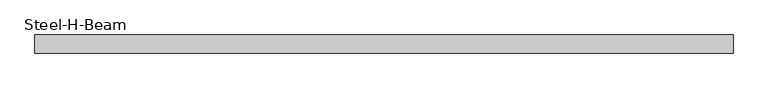
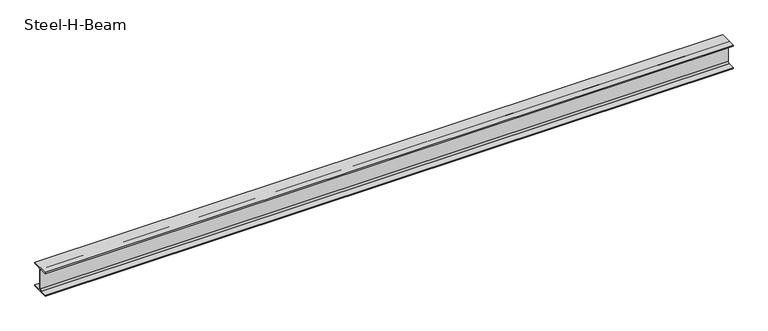
"""IFC4 building model written with IfcOpenShell, lengths in millimetres: beam geometry, Steel-H-Beam : BM121_H-244×175x7x11."""

import ifcopenshell
import ifcopenshell.guid

model = None  # the IFC model being written
_history = None  # IfcOwnerHistory: only IFC2X3 demands one
_inside = {}  # id of a spatial element -> (the spatial element, [elements in it])
_under = {}  # id of a project, library or spatial element -> (it, [spatial elements below it])
_declared = {}  # id of a project -> (the project, [libraries it declares])
_typed = {}  # id of a type object -> (the type object, [elements of that type])
_made_of = {}  # id of a material, layer set ... -> (it, [elements and type objects made of it])


def new_model(schema):
    """Start an empty IFC model of exactly this schema.

    Asked for "IFC4X3", IfcOpenShell would pick the latest addendum, in which some entities
    have other attributes; the version numbers below select the first issue.
    IFC2X3 requires an IfcOwnerHistory on every rooted entity: one is made here for all.
    """
    global model, _history
    if schema == "IFC4X3":
        model = ifcopenshell.file(schema_version=(4, 3, 0, 0))
    else:
        model = ifcopenshell.file(schema=schema)
    _inside.clear()
    _under.clear()
    _declared.clear()
    _typed.clear()
    _made_of.clear()
    _history = None
    if model.schema == "IFC2X3":
        org = make("IfcOrganization", Name="unknown")
        user = make(
            "IfcPersonAndOrganization",
            ThePerson=make("IfcPerson", FamilyName="unknown"),
            TheOrganization=org,
        )
        app = make(
            "IfcApplication",
            ApplicationDeveloper=org,
            Version="unknown",
            ApplicationFullName="unknown",
            ApplicationIdentifier="unknown",
        )
        _history = make(
            "IfcOwnerHistory",
            OwningUser=user,
            OwningApplication=app,
            ChangeAction="ADDED",
            CreationDate=0,
        )
    return model


def make(cls, **values):
    """One entity of the class cls with the attributes given. An attribute that is None is left unset."""
    return model.create_entity(
        cls, **{name: value for name, value in values.items() if value is not None}
    )


def rooted(cls, **values):
    """An entity with a GlobalId (a new one), such as an element, a storey or a relation."""
    return make(cls, GlobalId=ifcopenshell.guid.new(), OwnerHistory=_history, **values)


def si_unit(unit_type, name, prefix=None):
    """IfcSIUnit, for example si_unit("LENGTHUNIT", "METRE", prefix="MILLI")."""
    return make("IfcSIUnit", UnitType=unit_type, Prefix=prefix, Name=name)


def assignment(units):
    """IfcUnitAssignment: the units of a project."""
    return None if units is None else make("IfcUnitAssignment", Units=units)


def point(xyz):
    """IfcCartesianPoint."""
    return None if xyz is None else make("IfcCartesianPoint", Coordinates=xyz)


def direction(xyz):
    """IfcDirection."""
    return None if xyz is None else make("IfcDirection", DirectionRatios=xyz)


def frame(location, z_axis=None, x_axis=None):
    """IfcAxis2Placement3D, a coordinate frame: its origin and axes. An axis left out is left unset."""
    return make(
        "IfcAxis2Placement3D",
        Location=point(location),
        Axis=direction(z_axis),
        RefDirection=direction(x_axis),
    )


def frame_2d(location, x_axis=None):
    """IfcAxis2Placement2D, a coordinate frame in the plane: its origin and x axis."""
    return make(
        "IfcAxis2Placement2D", Location=point(location), RefDirection=direction(x_axis)
    )


def origin():
    """The frame at (0, 0, 0) with its axes left unset."""
    return frame((0.0, 0.0, 0.0))


def place(relative_to, where):
    """IfcLocalPlacement: puts the frame where relative to a parent placement (None: the world)."""
    return make(
        "IfcLocalPlacement", PlacementRelTo=relative_to, RelativePlacement=where
    )


def context(
    kind, dimensions, precision=None, world=None, true_north=None, identifier=None
):
    """IfcGeometricRepresentationContext, for example the 3D "Model" context."""
    return make(
        "IfcGeometricRepresentationContext",
        ContextIdentifier=identifier,
        ContextType=kind,
        CoordinateSpaceDimension=dimensions,
        Precision=precision,
        WorldCoordinateSystem=world,
        TrueNorth=true_north,
    )


def project(units=None, contexts=None):
    """IfcProject with its units and contexts."""
    return rooted(
        "IfcProject",
        Name="project",
        RepresentationContexts=contexts,
        UnitsInContext=assignment(units),
    )


def spatial(cls, under=None, at=None, **own):
    """A site, building, storey or space (cls), placed at a placement, below another one or the project."""
    s = rooted(cls, ObjectPlacement=at, **own)
    if under is not None:
        _under.setdefault(under.id(), (under, []))[1].append(s)
    return s


def polyline(points):
    """IfcPolyline through the points."""
    return make("IfcPolyline", Points=[point(p) for p in points])


def circle_curve(where, radius):
    """IfcCircle in the frame where."""
    return make("IfcCircle", Position=where, Radius=radius)


def trimmed(basis, trim1, trim2, sense, master):
    """IfcTrimmedCurve: the piece of a basis curve between two trims."""
    return make(
        "IfcTrimmedCurve",
        BasisCurve=basis,
        Trim1=trim1,
        Trim2=trim2,
        SenseAgreement=sense,
        MasterRepresentation=master,
    )


def segment(curve, same_sense, transition):
    """IfcCompositeCurveSegment."""
    return make(
        "IfcCompositeCurveSegment",
        Transition=transition,
        SameSense=same_sense,
        ParentCurve=curve,
    )


def composite_curve(segments, self_intersect=None):
    """IfcCompositeCurve: segments joined end to end."""
    return make("IfcCompositeCurve", Segments=segments, SelfIntersect=self_intersect)


def outline(outer, holes=None, kind="AREA"):
    """IfcArbitraryClosedProfileDef: a profile drawn as a closed curve; with holes, ...WithVoids."""
    if holes is None:
        return make("IfcArbitraryClosedProfileDef", ProfileType=kind, OuterCurve=outer)
    return make(
        "IfcArbitraryProfileDefWithVoids",
        ProfileType=kind,
        OuterCurve=outer,
        InnerCurves=holes,
    )


def extrude(swept, where, along, depth):
    """IfcExtrudedAreaSolid: the profile swept, set in the frame where, extruded along a direction by depth."""
    return make(
        "IfcExtrudedAreaSolid",
        SweptArea=swept,
        Position=where,
        ExtrudedDirection=direction(along),
        Depth=depth,
    )


def shape(context_of_items, identifier, shape_type, items):
    """IfcShapeRepresentation: the items that make up one representation, for example the "Body"."""
    return make(
        "IfcShapeRepresentation",
        ContextOfItems=context_of_items,
        RepresentationIdentifier=identifier,
        RepresentationType=shape_type,
        Items=items,
    )


def source(mapping_origin, context_of_items, identifier, shape_type, items):
    """IfcRepresentationMap: a shape defined once, which mapped items show again and again."""
    return make(
        "IfcRepresentationMap",
        MappingOrigin=mapping_origin,
        MappedRepresentation=shape(context_of_items, identifier, shape_type, items),
    )


def transform(
    local_origin,
    x_axis=None,
    y_axis=None,
    z_axis=None,
    scale=None,
    scale2=None,
    scale3=None,
    uniform=True,
):
    """IfcCartesianTransformationOperator3D, or its non-uniform kind. x_axis, y_axis, z_axis: its Axis1, 2, 3."""
    if uniform:
        return make(
            "IfcCartesianTransformationOperator3D",
            Axis1=direction(x_axis),
            Axis2=direction(y_axis),
            LocalOrigin=point(local_origin),
            Scale=scale,
            Axis3=direction(z_axis),
        )
    return make(
        "IfcCartesianTransformationOperator3DnonUniform",
        Axis1=direction(x_axis),
        Axis2=direction(y_axis),
        LocalOrigin=point(local_origin),
        Scale=scale,
        Axis3=direction(z_axis),
        Scale2=scale2,
        Scale3=scale3,
    )


def mapped(mapping_source, mapping_target):
    """IfcMappedItem: shows the shape of a source again, moved by a transform."""
    return make(
        "IfcMappedItem", MappingSource=mapping_source, MappingTarget=mapping_target
    )


def made_of(thing, what):
    """Note that an element or type object is made of a material, layer set ...; save() writes the relation."""
    if what is not None:
        _made_of.setdefault(what.id(), (what, []))[1].append(thing)
    return thing


def element(
    cls,
    number,
    at=None,
    inside=None,
    cuts=None,
    type_object=None,
    material=None,
    context=None,
    identifier="Body",
    shape_type=None,
    held_by="IfcProductDefinitionShape",
    body=None,
    shapes=None,
    **own,
):
    """One element of the class cls, such as IfcWall. Its Tag is "e" and its number.

    at: its placement. inside: the storey or other place that contains it. cuts: it is an
    opening in that element (IfcRelVoidsElement). A single representation is given by context,
    identifier, shape_type and body (its items); several are given by shapes. held_by: the class
    of the entity that holds the representations. save() writes the other relations.
    """
    e = rooted(cls, Tag="e%d" % number, ObjectPlacement=at, **own)
    if body is not None:
        shapes = [shape(context, identifier, shape_type, body)]
    if shapes is not None:
        e.Representation = make(held_by, Representations=shapes)
    if inside is not None:
        _inside.setdefault(inside.id(), (inside, []))[1].append(e)
    if cuts is not None:
        rooted(
            "IfcRelVoidsElement", RelatingBuildingElement=cuts, RelatedOpeningElement=e
        )
    if type_object is not None:
        _typed.setdefault(type_object.id(), (type_object, []))[1].append(e)
    return made_of(e, material)


def aggregate(whole, parts):
    """IfcRelAggregates: a whole, such as a stair, and the parts it consists of."""
    return rooted("IfcRelAggregates", RelatingObject=whole, RelatedObjects=parts)


def save(model, path):
    """Write the relations noted so far, then the file.

    IfcRelAggregates (storeys below a building ...), IfcRelContainedInSpatialStructure (elements
    in a storey), IfcRelDefinesByType, IfcRelAssociatesMaterial and IfcRelDeclares: one each for
    every whole, place, type object, material and project.
    """
    for whole, parts in _under.values():
        aggregate(whole, parts)
    for where, things in _inside.values():
        rooted(
            "IfcRelContainedInSpatialStructure",
            RelatedElements=things,
            RelatingStructure=where,
        )
    for kind, things in _typed.values():
        rooted("IfcRelDefinesByType", RelatedObjects=things, RelatingType=kind)
    for what, things in _made_of.values():
        rooted("IfcRelAssociatesMaterial", RelatedObjects=things, RelatingMaterial=what)
    for by, libraries in _declared.values():
        rooted("IfcRelDeclares", RelatingContext=by, RelatedDefinitions=libraries)
    model.write(path)


def steel_h_beam_22148b76(model_context):
    return source(origin(), model_context, "Body", "SweptSolid", [
        extrude(outline(composite_curve([segment(polyline([(87.5, -111.0), (87.5, -122.0), (-87.5, -122.0), (-87.5, -111.0), (-19.5, -111.0)]), True, "CONTINUOUS"), segment(trimmed(circle_curve(frame_2d((-19.5, -95.0)), 16.0), [point((-19.5, -111.0))], [point((-3.5, -95.0))], True, "CARTESIAN"), True, "CONTINUOUS"), segment(polyline([(-3.5, -95.0), (-3.5, 95.0)]), True, "CONTINUOUS"), segment(trimmed(circle_curve(frame_2d((-19.5, 95.0)), 16.0), [point((-3.5, 95.0))], [point((-19.5, 111.0))], True, "CARTESIAN"), True, "CONTINUOUS"), segment(polyline([(-19.5, 111.0), (-87.5, 111.0), (-87.5, 122.0), (87.5, 122.0), (87.5, 111.0), (19.5, 111.0)]), True, "CONTINUOUS"), segment(trimmed(circle_curve(frame_2d((19.5, 95.0)), 16.0), [point((19.5, 111.0))], [point((3.5, 95.0))], True, "CARTESIAN"), True, "CONTINUOUS"), segment(polyline([(3.5, 95.0), (3.5, -95.0)]), True, "CONTINUOUS"), segment(trimmed(circle_curve(frame_2d((19.5, -95.0)), 16.0), [point((3.5, -95.0))], [point((19.5, -111.0))], True, "CARTESIAN"), True, "CONTINUOUS"), segment(polyline([(19.5, -111.0), (87.5, -111.0)]), True, "CONTINUOUS")], self_intersect=False)), frame((-3361.8243373, 0.0, 0.0), z_axis=(1.0, 0.0, 0.0), x_axis=(0.0, 1.0, 0.0)), (0.0, 0.0, 1.0), 6724.6),
    ])


if __name__ == "__main__":
    model = new_model("IFC4")
    model_context = context("Model", 3, world=origin())
    ifc_project = project(units=[si_unit("LENGTHUNIT", "METRE", prefix="MILLI")], contexts=[model_context])
    site = spatial("IfcSite", under=ifc_project)
    building = spatial("IfcBuilding", under=site)
    placement = place(None, origin())
    steel_h_beam_shape = steel_h_beam_22148b76(model_context)
    element("IfcBeam", 1, ObjectType="Steel-H-Beam : BM121_H-244×175x7x11", at=placement, inside=building, context=model_context, shape_type="MappedRepresentation", body=[
        mapped(steel_h_beam_shape, transform((0.0, 0.0, 0.0), x_axis=(1.0, 0.0, 0.0), y_axis=(0.0, 1.0, 0.0), z_axis=(0.0, 0.0, 1.0))),
    ])
    save(model, "model.ifc")

# Revit data of these elements
# Type "Steel-H-Beam : BM121_H-244×175x7x11"
#   Surface Area = 1.14653 m²/m
#   Section Area = 56.2375 cm²
#   Mass per Unit Length = 44.1465 kg/m
#   Length [instance default] = 3000 mm
#   B = 175 mm
#   H = 244 mm
#   r = 16 mm
#   tw = 7 mm
#   tf = 11 mm
#   hec_material4 [instance default] = none
#   hec_material3 [instance default] = none
#   hec_material2 [instance default] = none
#   hec_material1 [instance default] = none
#   Structural Material [instance default] = Steel, 45-345
#   Assembly Code = ""
# Element 1 (IfcBeam, "Steel-H-Beam : BM121_H-244×175x7x11")
#   hec_material3 = F01AC000-00002_Building/Shelter Fire Proofing Work_Intumescent Coating Type_1 hr. rating (UL 1709))
#   hec_material2 = S01AA010-00002_Main Steel Structure Fabrication Work_Shelter/Building_Steel Painting/Coating_for Fireproofed Steel Surface, Surface Preparation & Primer Coat
#   hec_material1 = S03AA028-00001_Main Steel Structure Erection Work_Shelter/Building_Medium Steel
#   Materials on its faces: "Steel, 45-345"
# Materials
#   "Steel, 45-345": class "Metal", colour RGB 189 187 185, transparency 0, Description = "Steel 345 MPa", Cost = 0
#   "F01AC000-00002_Building/Shelter Fire Proofing Work_Intumescent Coating Type_1 hr. rating (UL 1709))": class "Metal", colour RGB 255 128 128, transparency 0, Description = "Paint finished steel", W00) Work Master Code = "F01AC000-00002", W01) Work Master_Lv1 = "Building/Shelter Fire Proofing Work", W02) Work Master_Lv2 = "Intumescent Coating Type", W03) Work Master_Spec.1 = "1 hr. rating (UL 1709)", Cost = 0
#   "S01AA010-00002_Main Steel Structure Fabrication Work_Shelter/Building_Steel Painting/Coating_for Fireproofed Steel Surface, Surface Preparation & Primer Coat": class "Metal", colour RGB 120 120 120, transparency 0, Description = "Paint finished steel", W00) Work Master Code = "SS01AA010-00002", W01) Work Master_Lv1 = "Main Steel Structure Fabrication Work", W02) Work Master_Lv2 = "Shelter/Building", W03) Work Master_Spec.1 = "Steel Painting/Coating", W04) Work Master_Spec.2 = "for Fireproofed Steel Surface, Surface Preparation & Primer Coat", Cost = 0
#   "S03AA028-00001_Main Steel Structure Erection Work_Shelter/Building_Medium Steel": class "Metal", colour RGB 120 120 120, transparency 0, Comments = "(90KG/M>Weight≥30KG/M)", Description = "Structural steel 50ksi", W00) Work Master Code = "S03AA028-0001", W01) Work Master_Lv1 = "Main Steel Structure Erection Work", W02) Work Master_Lv2 = "Shelter/Building", W03) Work Master_Spec.1 = "Medium Steel (90KG/M>Weight≥30KG/M)", Cost = 0
